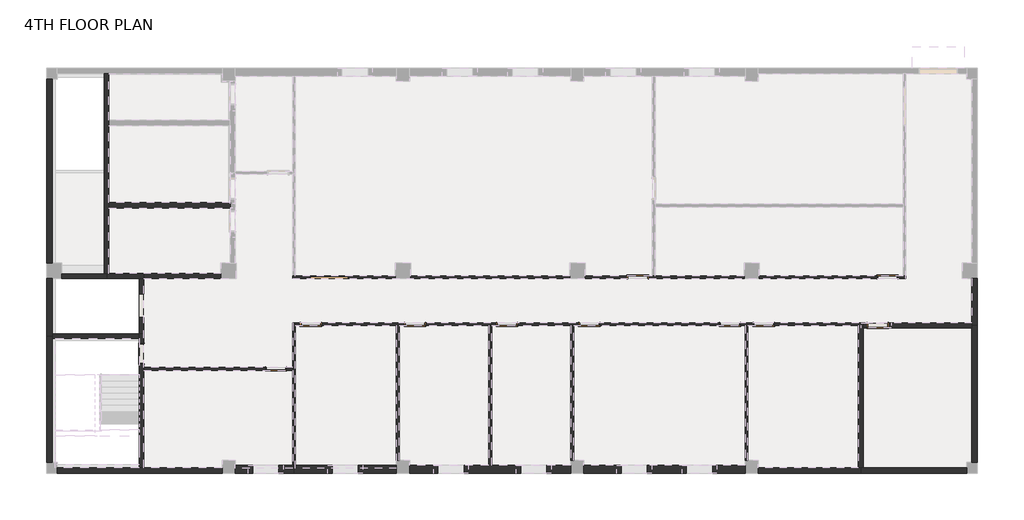
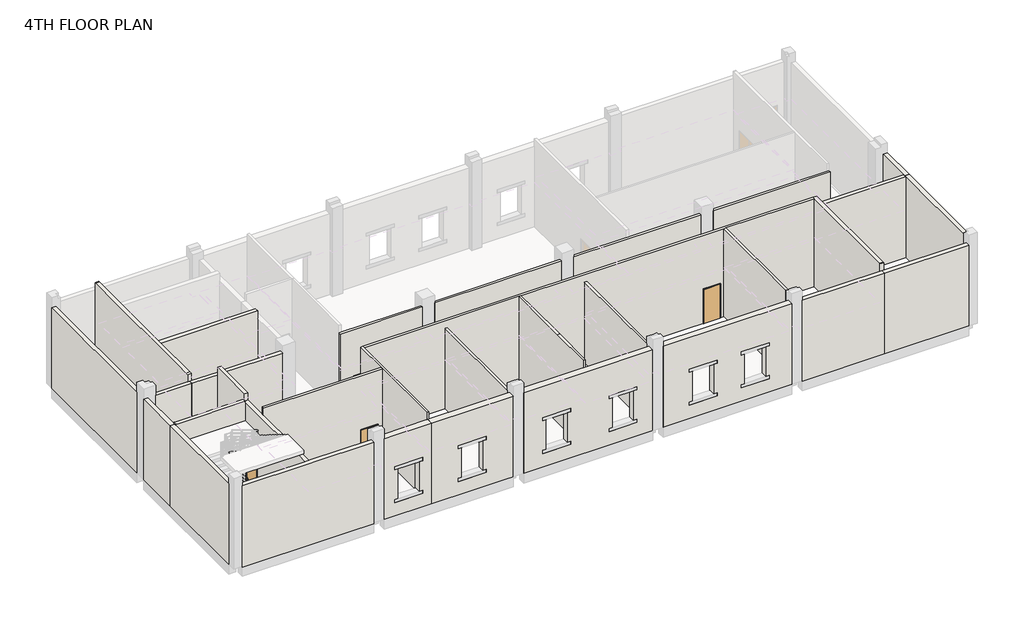
# One storey, part 1 of 6: 34 walls, 12 doors.
# Revit data of these elements (continued)
# Type "DR110-Single Door : DR111-Steel Door-1000x2100mm"
#   Description = "DSDSSD"
#   Type Mark = "SD"
#   Analytic Construction = "<None>"
#   프레임 투영 외부. = 25 mm
#   프레임 투영 내부. = 25 mm
#   프레임 폭 = 75 mm
#   Height = 2100 mm
#   Width = 1000 mm
#   Define Thermal Properties by = 1
#   문 패널 = SD1 문 패널
#   문 프레임 = A04AQ098-00002_Steel Door_non FP_single
#   Function = (empty or 0)
#   Wall Closure = (empty or 0)
# Type "DR110-Single Door : DR112-Steel Door-1000x2100mm_Panic Bar"
#   Type Mark = "SD"
#   Analytic Construction = "<None>"
#   프레임 투영 외부. = 25 mm
#   프레임 투영 내부. = 25 mm
#   프레임 폭 = 75 mm
#   Height = 2100 mm
#   Width = 1000 mm
#   Define Thermal Properties by = 1
#   문 패널 = SD1 문 패널
#   문 프레임 = A04AQ098-00002_Steel Door_non FP_single
#   Function = (empty or 0)
#   Wall Closure = (empty or 0)
# Type "DR120-Double Door : DR121-Steel Door-2000x2100mm"
#   Type Mark = "SD"
#   프레임 = ""
#   철물 = ""
#   유리/마감 = ""
#   위치/개소 = ""
#   부호 = "1/SD"
#   문번호 = ""
#   문기호 = "SD"
#   Analytic Construction = "<None>"
#   Height = 2100 mm
#   Width = 1800 mm
#   Define Thermal Properties by = 1
#   문 틀 = A04AQ098-00003_Steel Door_non FP_double
#   문 = 문
#   Function = (empty or 0)
#   Assembly Code = ""
#   Wall Closure = (empty or 0)
# Type "WA120_Ext. RC Wall_AG_300- W1(2)"
#   Type Comments = ""
#   Type Mark = "W1"
#   Layers, outside or top first: 1 mm "A04AL077-00001_Ext Wall Painting_Acrylic Emulsion Paint" (function 4); 250 mm "A03AD032-00007_Structural Concrete_25MPa-30MPa" (function 1); 0 mm "A03AD036-00001_Form Work (1 time in use)" (function 100)
# Type "WA120_Ext. RC Wall_AG_300- W1(1)"
#   Type Comments = ""
#   Type Mark = "W1"
#   Layers, outside or top first: 1 mm "A04AL077-00001_Ext Wall Painting_Acrylic Emulsion Paint" (function 4); 250 mm "A03AD032-00007_Structural Concrete_25MPa-30MPa" (function 1); 0 mm "A03AD036-00001_Form Work (1 time in use)" (function 100); 1 mm "A04AL078-00002_Int Wall Painting_Water Emulsion Paint" (function 5); 0 mm "A04AL081-00007_Skirt_Epoxy Paint" (function 100)
# Type "WA120_Ext. RC Wall_AG_300- W1(3)"
#   Type Comments = ""
#   Type Mark = "W1"
#   Layers, outside or top first: 1 mm "A04AL077-00001_Ext Wall Painting_Acrylic Emulsion Paint" (function 4); 250 mm "A03AD032-00007_Structural Concrete_25MPa-30MPa" (function 1); 0 mm "A03AD036-00001_Form Work (1 time in use)" (function 100); 1 mm "A04AL078-00002_Int Wall Painting_Water Emulsion Paint" (function 5); 0 mm "A04AM084-00013_Skirt_Vinyl Tile w/Mortar Bond Coat or Adhesive" (function 100)
# Type "WA140_Int. RC Wall_200- W2"
#   Type Comments = ""
#   Type Mark = "W2"
#   Layers, outside or top first: 200 mm "A03AD032-00007_Structural Concrete_25MPa-30MPa" (function 1)
# Type "WAFC221_Int. Brick Wall_200_7"
#   Type Comments = ""
#   Layers, outside or top first: 190 mm "A04AK073-00002_Concrete Brick_1.0B" (function 1); 0 mm "A04AN085-00001_Liquid Waterproofing" (function 100); 21 mm "A04AS164-00002_Plastering_Int" (function 2); 9 mm "A04AM082-00002_Wall Tile_Glazed ceramic tile w/Mortar Bond Coat or Adhesive" (function 5)
# Type "WAFC221_Int. Brick Wall_200_1"
#   Type Comments = ""
#   Layers, outside or top first: 0 mm "A04AL081-00002_Skirt_Epoxy Paint" (function 100); 1 mm "A04AL078-00002_Int Wall Painting_Water Emulsion Paint" (function 4); 15 mm "A04AS164-00002_Plastering_Int" (function 2); 190 mm "A04AK073-00002_Concrete Brick_1.0B" (function 1); 15 mm "A04AS164-00002_Plastering_Int" (function 2); 1 mm "A04AL078-00002_Int Wall Painting_Water Emulsion Paint" (function 5); 0 mm "A04AM084-00013_Skirt_Vinyl Tile w/Mortar Bond Coat or Adhesive" (function 100)
# Type "WAFC221_Int. Brick Wall_200_8"
#   Type Comments = ""
#   Layers, outside or top first: 9 mm "A04AM082-00002_Wall Tile_Glazed ceramic tile w/Mortar Bond Coat or Adhesive" (function 4); 21 mm "A04AS164-00002_Plastering_Int" (function 2); 0 mm "A04AN085-00001_Liquid Waterproofing" (function 100); 190 mm "A04AK073-00002_Concrete Brick_1.0B" (function 1); 0 mm "A04AN085-00001_Liquid Waterproofing" (function 100); 21 mm "A04AS164-00002_Plastering_Int" (function 2); 9 mm "A04AM082-00002_Wall Tile_Glazed ceramic tile w/Mortar Bond Coat or Adhesive" (function 5)
# Type "WAFC221_Int. Brick Wall_200_6"
#   Type Comments = ""
#   Layers, outside or top first: 0 mm "A04AM084-00013_Skirt_Vinyl Tile w/Mortar Bond Coat or Adhesive" (function 100); 1 mm "A04AL078-00002_Int Wall Painting_Water Emulsion Paint" (function 4); 15 mm "A04AS164-00002_Plastering_Int" (function 2); 190 mm "A04AK073-00002_Concrete Brick_1.0B" (function 1); 0 mm "A04AN085-00001_Liquid Waterproofing" (function 100); 21 mm "A04AS164-00002_Plastering_Int" (function 2); 9 mm "A04AM082-00002_Wall Tile_Glazed ceramic tile w/Mortar Bond Coat or Adhesive" (function 5)
# Type "WA140_Int. RC Wall_200- W2(1)"
#   Type Comments = ""
#   Type Mark = "W2"
#   Layers, outside or top first: 0 mm "A04AM084-00013_Skirt_Vinyl Tile w/Mortar Bond Coat or Adhesive" (function 100); 1 mm "A04AL078-00002_Int Wall Painting_Water Emulsion Paint" (function 4); 200 mm "A03AD032-00007_Structural Concrete_25MPa-30MPa" (function 1); 0 mm "A03AD036-00001_Form Work (1 time in use)" (function 100); 1 mm "A04AL078-00002_Int Wall Painting_Water Emulsion Paint" (function 4); 0 mm "A04AM084-00013_Skirt_Vinyl Tile w/Mortar Bond Coat or Adhesive" (function 100)
# Type "WA140_Int. RC Wall_200- W2(3)"
#   Type Comments = ""
#   Type Mark = "W2"
#   Layers, outside or top first: 200 mm "A03AD032-00007_Structural Concrete_25MPa-30MPa" (function 1); 0 mm "A03AD036-00001_Form Work (1 time in use)" (function 100); 1 mm "A04AL078-00002_Int Wall Painting_Water Emulsion Paint" (function 4); 0 mm "A04AL081-00007_Skirt_Epoxy Paint" (function 100)
# Type "WA140_Int. RC Wall_200- W2(2)"
#   Type Comments = ""
#   Type Mark = "W2"
#   Layers, outside or top first: 200 mm "A03AD032-00007_Structural Concrete_25MPa-30MPa" (function 1); 0 mm "A03AD036-00001_Form Work (1 time in use)" (function 100); 1 mm "A04AL078-00002_Int Wall Painting_Water Emulsion Paint" (function 4); 0 mm "A04AM084-00013_Skirt_Vinyl Tile w/Mortar Bond Coat or Adhesive" (function 100)
# Type "WAFC356 Interior-WF-Ceramic Tile"
#   Type Comments = ""
#   Layers, outside or top first: 0 mm "A04AN085-00001_Liquid Waterproofing" (function 100); 21 mm "A04AS164-00002_Plastering_Int" (function 2); 9 mm "A04AM082-00002_Wall Tile_Glazed ceramic tile w/Mortar Bond Coat or Adhesive" (function 4)
# Type "WA452_Int. Gypsum Wall 2 Layer_2 Hr_125"
#   Type Comments = ""
#   Layers, outside or top first: 0 mm "A04AM084-00013_Skirt_Vinyl Tile w/Mortar Bond Coat or Adhesive" (function 100); 0 mm "A04AL078-00002_Int Wall Painting_Water Emulsion Paint" (function 100); 125 mm "A04AR143-00010_Gypsumboard Partition Wall_THK 12.5mm 2ply_Mineral wool" (function 2); 0 mm "A04AL078-00002_Int Wall Painting_Water Emulsion Paint" (function 100); 0 mm "A04AM084-00013_Skirt_Vinyl Tile w/Mortar Bond Coat or Adhesive" (function 100)
# Type "WAF310_Ext. Cavity Wall Brick_90_50_190_1"
#   Type Comments = ""
#   Layers, outside or top first: 1 mm "A04AL077-00001_Ext Wall Painting_Acrylic Emulsion Paint" (function 4); 20 mm "A04AS164-00001_Plastering_Ext" (function 2); 90 mm "A04AK073-00001_Concrete Brick_0.5B" (function 1); 50 mm "A04AK076-00001_Mineral Wool_THK 50-75mm" (function 3); 190 mm "A04AK073-00002_Concrete Brick_1.0B" (function 1); 15 mm "A04AS164-00002_Plastering_Int" (function 2); 1 mm "A04AL078-00002_Int Wall Painting_Water Emulsion Paint" (function 4); 0 mm "A04AL081-00007_Skirt_Epoxy Paint" (function 100)
# Type "WAF310_Ext. Cavity Wall Brick_90_50_190_2"
#   Type Comments = ""
#   Layers, outside or top first: 1 mm "A04AL077-00001_Ext Wall Painting_Acrylic Emulsion Paint" (function 4); 20 mm "A04AS164-00001_Plastering_Ext" (function 2); 90 mm "A04AK073-00001_Concrete Brick_0.5B" (function 1); 50 mm "A04AK076-00001_Mineral Wool_THK 50-75mm" (function 3); 190 mm "A04AK073-00002_Concrete Brick_1.0B" (function 1); 15 mm "A04AS164-00002_Plastering_Int" (function 2); 1 mm "A04AL078-00002_Int Wall Painting_Water Emulsion Paint" (function 4); 0 mm "A04AM084-00013_Skirt_Vinyl Tile w/Mortar Bond Coat or Adhesive" (function 100)
# Elements 1, 2, 3, 4, 5, 6, 7, 8, 9, 10 (IfcDoor, "DR110-Single Door : DR111-Steel Door-1000x2100mm")
#   Head = "1"
#   Jamb = "2"
#   Sill = "5"
#   Door Type = "A"
#   Phase Created = New Construction
#   Materials on its faces: "A04AQ098-00002_Steel Door_non FP_single", "SD1 문 패널"
# Element 11 (IfcDoor, "DR110-Single Door : DR112-Steel Door-1000x2100mm_Panic Bar")
#   Head = "1"
#   Jamb = "2"
#   Sill = "3"
#   Door Type = "A"
#   Phase Created = New Construction
#   Materials on its faces: "A04AQ098-00002_Steel Door_non FP_single", "SD1 문 패널"
# Element 12 (IfcDoor, "DR120-Double Door : DR121-Steel Door-2000x2100mm")
#   Head = "1"
#   Jamb = "2"
#   Sill = "5"
#   Door Type = "B"
#   FLOOR = "4TH FLOOR PLAN"
#   Phase Created = New Construction
#   Materials on its faces: "A04AQ098-00003_Steel Door_non FP_double", "문"
# Element 13 (IfcWall, "WA120_Ext. RC Wall_AG_300- W1(2)")
#   Top Offset = -600 mm
#   Base Offset = 0 mm
#   wall height = 4900 mm
#   Phase Created = New Construction
#   Base Constraint = 4TH FLOOR PLAN
#   Top Constraint = ROOF PLAN
#   Materials on its faces: "Default Wall", "A04AL077-00001_Ext Wall Painting_Acrylic Emulsion Paint", "A03AD032-00007_Structural Concrete_25MPa-30MPa"
# Elements 14, 29 (IfcWall, "WA120_Ext. RC Wall_AG_300- W1(1)")
#   Top Offset = -600 mm
#   Base Offset = 0 mm
#   wall height = 4900 mm
#   Phase Created = New Construction
#   Base Constraint = 4TH FLOOR PLAN
#   Top Constraint = ROOF PLAN
#   Materials on its faces: "Default Wall", "A04AL077-00001_Ext Wall Painting_Acrylic Emulsion Paint", "A04AL078-00002_Int Wall Painting_Water Emulsion Paint"
# Element 15 (IfcWall, "WA120_Ext. RC Wall_AG_300- W1(3)")
#   Top Offset = -600 mm
#   Base Offset = 0 mm
#   wall height = 4900 mm
#   Phase Created = New Construction
#   Base Constraint = 4TH FLOOR PLAN
#   Top Constraint = ROOF PLAN
#   Materials on its faces: "Default Wall", "A04AL078-00002_Int Wall Painting_Water Emulsion Paint", "A04AL077-00001_Ext Wall Painting_Acrylic Emulsion Paint"
# Element 16 (IfcWall, "WA140_Int. RC Wall_200- W2")
#   built-in parameter 1001111 = -50 mm
#   Top Offset = -600 mm
#   Base Offset = -50 mm
#   wall height = 4950 mm
#   Phase Created = New Construction
#   Base Constraint = 4TH FLOOR PLAN
#   Top Constraint = ROOF PLAN
#   Materials on its faces: "A03AD032-00007_Structural Concrete_25MPa-30MPa", "A04AL078-00002_Int Wall Painting_Water Emulsion Paint"
# Element 17 (IfcWall, "WAFC221_Int. Brick Wall_200_7")
#   built-in parameter 1001111 = -50 mm
#   Top Offset = -150 mm
#   Base Offset = -50 mm
#   wall height = 5400 mm
#   Phase Created = New Construction
#   Base Constraint = 4TH FLOOR PLAN
#   Top Constraint = ROOF PLAN
#   Materials on its faces: "Default Wall", "A04AM082-00002_Wall Tile_Glazed ceramic tile w/Mortar Bond Coat or Adhesive", "A04AK073-00002_Concrete Brick_1.0B"
# Element 18 (IfcWall, "WAFC221_Int. Brick Wall_200_1")
#   built-in parameter 1001111 = -50 mm
#   Top Offset = -150 mm
#   Base Offset = -50 mm
#   wall height = 5400 mm
#   Phase Created = New Construction
#   Base Constraint = 4TH FLOOR PLAN
#   Top Constraint = ROOF PLAN
#   Materials on its faces: "Default Wall", "A04AL078-00002_Int Wall Painting_Water Emulsion Paint"
# Element 19 (IfcWall, "WAFC221_Int. Brick Wall_200_1")
#   built-in parameter 1001111 = -50 mm
#   Top Offset = -600 mm
#   Base Offset = -50 mm
#   wall height = 4950 mm
#   Phase Created = New Construction
#   Base Constraint = 4TH FLOOR PLAN
#   Top Constraint = ROOF PLAN
#   Materials on its faces: "Default Wall", "A04AL078-00002_Int Wall Painting_Water Emulsion Paint"
# Element 20 (IfcWall, "WAFC221_Int. Brick Wall_200_8")
#   built-in parameter 1001111 = -50 mm
#   Top Offset = -150 mm
#   Base Offset = -50 mm
#   wall height = 5400 mm
#   Phase Created = New Construction
#   Base Constraint = 4TH FLOOR PLAN
#   Top Constraint = ROOF PLAN
#   Materials on its faces: "Default Wall", "A04AM082-00002_Wall Tile_Glazed ceramic tile w/Mortar Bond Coat or Adhesive"
# Element 21 (IfcWall, "WAFC221_Int. Brick Wall_200_6")
#   Top Offset = -600 mm
#   Base Offset = 0 mm
#   wall height = 4900 mm
#   Phase Created = New Construction
#   Base Constraint = 4TH FLOOR PLAN
#   Top Constraint = ROOF PLAN
#   Materials on its faces: "Default Wall", "A04AM082-00002_Wall Tile_Glazed ceramic tile w/Mortar Bond Coat or Adhesive", "A04AL078-00002_Int Wall Painting_Water Emulsion Paint"
# Element 22 (IfcWall, "WA120_Ext. RC Wall_AG_300- W1(3)")
#   built-in parameter 1001111 = -50 mm
#   Top Offset = -600 mm
#   Base Offset = -50 mm
#   wall height = 4950 mm
#   Phase Created = New Construction
#   Base Constraint = 4TH FLOOR PLAN
#   Top Constraint = ROOF PLAN
#   Materials on its faces: "Default Wall", "A04AL077-00001_Ext Wall Painting_Acrylic Emulsion Paint", "A04AL078-00002_Int Wall Painting_Water Emulsion Paint"
# Element 23 (IfcWall, "WA120_Ext. RC Wall_AG_300- W1(1)")
#   Top Offset = -600 mm
#   Base Offset = 0 mm
#   wall height = 4900 mm
#   Phase Created = New Construction
#   Base Constraint = 4TH FLOOR PLAN
#   Top Constraint = ROOF PLAN
#   Materials on its faces: "Default Wall", "A04AL078-00002_Int Wall Painting_Water Emulsion Paint", "A04AL077-00001_Ext Wall Painting_Acrylic Emulsion Paint"
# Element 24 (IfcWall, "WA140_Int. RC Wall_200- W2(1)")
#   built-in parameter 1001111 = -50 mm
#   Top Offset = -600 mm
#   Base Offset = -50 mm
#   wall height = 4950 mm
#   Phase Created = New Construction
#   Base Constraint = 4TH FLOOR PLAN
#   Top Constraint = ROOF PLAN
#   Materials on its faces: "Default Wall", "A04AL078-00002_Int Wall Painting_Water Emulsion Paint", "A03AD032-00007_Structural Concrete_25MPa-30MPa"
# Element 25 (IfcWall, "WA140_Int. RC Wall_200- W2(3)")
#   built-in parameter 1001111 = -50 mm
#   Top Offset = -550 mm
#   Base Offset = -50 mm
#   wall height = 5000 mm
#   Phase Created = New Construction
#   Base Constraint = 4TH FLOOR PLAN
#   Top Constraint = ROOF PLAN
#   Materials on its faces: "Default Wall", "A04AL078-00002_Int Wall Painting_Water Emulsion Paint", "A03AD032-00007_Structural Concrete_25MPa-30MPa"
# Element 26 (IfcWall, "WA140_Int. RC Wall_200- W2(2)")
#   Comments = ""
#   built-in parameter 1001111 = -50 mm
#   Top Offset = -150 mm
#   Base Offset = -50 mm
#   wall height = 5400 mm
#   Phase Created = New Construction
#   Base Constraint = 4TH FLOOR PLAN
#   Top Constraint = ROOF PLAN
#   Materials on its faces: "Default Wall", "A04AL078-00002_Int Wall Painting_Water Emulsion Paint", "A03AD032-00007_Structural Concrete_25MPa-30MPa"
# Element 27 (IfcWall, "WA140_Int. RC Wall_200- W2")
#   built-in parameter 1001111 = -50 mm
#   Top Offset = -600 mm
#   Base Offset = -50 mm
#   wall height = 4950 mm
#   Phase Created = New Construction
#   Base Constraint = 4TH FLOOR PLAN
#   Top Constraint = ROOF PLAN
#   Materials on its faces: "A03AD032-00007_Structural Concrete_25MPa-30MPa"
# Element 28 (IfcWall, "WA120_Ext. RC Wall_AG_300- W1(3)")
#   Top Offset = -600 mm
#   Base Offset = 0 mm
#   wall height = 4900 mm
#   Phase Created = New Construction
#   Base Constraint = 4TH FLOOR PLAN
#   Top Constraint = ROOF PLAN
#   Materials on its faces: "Default Wall", "A04AL077-00001_Ext Wall Painting_Acrylic Emulsion Paint", "A04AL078-00002_Int Wall Painting_Water Emulsion Paint"
# Element 30 (IfcWall, "WAFC356 Interior-WF-Ceramic Tile")
#   Top Offset = 0 mm
#   Base Offset = 0 mm
#   Unconnected Height = 3000 mm
#   wall height = 3000 mm
#   Phase Created = New Construction
#   Base Constraint = 4TH FLOOR PLAN
#   Materials on its faces: "Default Wall", "A04AM082-00002_Wall Tile_Glazed ceramic tile w/Mortar Bond Coat or Adhesive", "A04AS164-00002_Plastering_Int"
# Element 31 (IfcWall, "WA120_Ext. RC Wall_AG_300- W1(2)")
#   Comments = ""
#   Top Offset = -600 mm
#   Base Offset = 0 mm
#   wall height = 4900 mm
#   Phase Created = New Construction
#   Base Constraint = 4TH FLOOR PLAN
#   Top Constraint = ROOF PLAN
#   Materials on its faces: "Default Wall", "A04AL077-00001_Ext Wall Painting_Acrylic Emulsion Paint", "A03AD032-00007_Structural Concrete_25MPa-30MPa"
# Elements 32, 36, 37, 38, 39, 40 (IfcWall, "WA452_Int. Gypsum Wall 2 Layer_2 Hr_125")
#   Top Offset = -600 mm
#   Base Offset = 0 mm
#   wall height = 4900 mm
#   Phase Created = New Construction
#   Base Constraint = 4TH FLOOR PLAN
#   Top Constraint = ROOF PLAN
#   Materials on its faces: "Default Wall", "A04AR143-00010_Gypsumboard Partition Wall_THK 12.5mm 2ply_Mineral wool"
# Elements 33, 34, 35, 42 (IfcWall, "WA452_Int. Gypsum Wall 2 Layer_2 Hr_125")
#   Top Offset = -150 mm
#   Base Offset = 0 mm
#   wall height = 5350 mm
#   Phase Created = New Construction
#   Base Constraint = 4TH FLOOR PLAN
#   Top Constraint = ROOF PLAN
#   Materials on its faces: "Default Wall", "A04AR143-00010_Gypsumboard Partition Wall_THK 12.5mm 2ply_Mineral wool"
# Element 41 (IfcWall, "WA452_Int. Gypsum Wall 2 Layer_2 Hr_125")
#   Top Offset = -150 mm
#   Base Offset = 0 mm
#   wall height = 5350 mm
#   Phase Created = New Construction
#   Base Constraint = 4TH FLOOR PLAN
#   Top Constraint = ROOF PLAN
#   Materials on its faces: "A04AR143-00010_Gypsumboard Partition Wall_THK 12.5mm 2ply_Mineral wool", "Default Wall"
# Element 43 (IfcWall, "WAF310_Ext. Cavity Wall Brick_90_50_190_1")
#   Top Offset = -600 mm
#   Base Offset = 0 mm
#   wall height = 4900 mm
#   Phase Created = New Construction
#   Base Constraint = 4TH FLOOR PLAN
#   Top Constraint = ROOF PLAN
#   Materials on its faces: "Default Wall", "A04AL077-00001_Ext Wall Painting_Acrylic Emulsion Paint", "A04AL078-00002_Int Wall Painting_Water Emulsion Paint"
# Elements 44, 45, 46 (IfcWall, "WAF310_Ext. Cavity Wall Brick_90_50_190_2")
#   Top Offset = -600 mm
#   Base Offset = 0 mm
#   wall height = 4900 mm
#   Phase Created = New Construction
#   Base Constraint = 4TH FLOOR PLAN
#   Top Constraint = ROOF PLAN
#   Materials on its faces: "Default Wall", "A04AL077-00001_Ext Wall Painting_Acrylic Emulsion Paint", "A04AL078-00002_Int Wall Painting_Water Emulsion Paint"
# Materials
#   "SD1 문 패널": class "금속", colour RGB 247 247 247, transparency 0, Description = "STEEL DOOR (1000Wx2100H)"
#   "A04AQ098-00002_Steel Door_non FP_single": class "금속", colour RGB 247 247 247, transparency 0, Description = "Steel Door", W00) Work Master Code = "A04AQ098-00002", W01) Work Master_Lv1 = "Finishing Work", W02) Work Master_Lv2 = "Door & Window Work", W03) Work Master_Spec.1 = "Steel Door w/ Steel Frame", W04) Work Master_Spec.2 = "Fire Protective Rating: N/A, Single Door", W05) Work Master_Spec.3 = "w/ Hardware & Accessories", Cost = 0
#   "A04AQ098-00003_Steel Door_non FP_double": class "금속", colour RGB 247 247 247, transparency 0, Description = "Steel Door", W00) Work Master Code = "A04AQ098-00003", W01) Work Master_Lv1 = "Finishing Work", W02) Work Master_Lv2 = "Door & Window Work", W03) Work Master_Spec.1 = "Steel Door w/ Steel Frame", W04) Work Master_Spec.2 = "Fire Protective Rating: N/A, Double Door", W05) Work Master_Spec.3 = "w/ Hardware & Accessories", Cost = 0
#   "문": class "다양한", colour RGB 247 247 247, transparency 0
#   "A04AL077-00001_Ext Wall Painting_Acrylic Emulsion Paint": class "Finish", colour RGB 128 128 64, transparency 0, Description = "ACRYLIC EMULSION PAINT", W00) Work Master Code = "A04AL077-00001", W01) Work Master_Lv1 = "Finishing Work", W02) Work Master_Lv2 = "Painting Work", W03) Work Master_Spec.1 = "External Wall Painting", W04) Work Master_Spec.2 = "Acrylic Emulsion Paint", Cost = 0
#   "A03AD032-00007_Structural Concrete_25MPa-30MPa": class "Concrete", colour RGB 176 176 176, transparency 0, Keynote = "09910.A1", Description = "ACRYLIC EMULSION PAINT ON\nFAIR FACED CONC.", W00) Work Master Code = "A03AD032-00007", W01) Work Master_Lv1 = "Concrete Work", W02) Work Master_Lv2 = "Superstructure Work", W03) Work Master_Spec.1 = "Structural Concrete", W04) Work Master_Spec.2 = "Cement Type-1", W05) Work Master_Spec.3 = "25MPa < F'c (Cylinder Strength) ≤ 30MPa", Cost = 0
#   "A03AD036-00001_Form Work (1 time in use)": class "Wood", colour RGB 149 120 74, transparency 0, Description = "Plywood", W00) Work Master Code = "A03AD036-00001", W01) Work Master_Lv1 = "Concrete Work", W02) Work Master_Lv2 = "Superstructure Work", W03) Work Master_Spec.1 = "Form Work (1 time in use)", W04) Work Master_Spec.2 = "Flat Form", W05) Work Master_Spec.3 = "Dressed Lumber, Plywood or Steel Form(Wood Planks are not Allowed) incl. Chamfer", Cost = 0
#   "A04AL078-00002_Int Wall Painting_Water Emulsion Paint": class "Finish", colour RGB 128 128 64, transparency 0, Description = "WATER EMULSION PAINT", W00) Work Master Code = "A04AL078-00002", W01) Work Master_Lv1 = "Finishing Work", W02) Work Master_Lv2 = "Painting Work", W03) Work Master_Spec.1 = "Internal Wall Painting", W04) Work Master_Spec.2 = "Water Emulsion Paint", Cost = 0
#   "A04AL081-00007_Skirt_Epoxy Paint": class "Finish", colour RGB 128 128 64, transparency 0, Description = "플라스틱", W00) Work Master Code = "A04AL081-00007", W01) Work Master_Lv1 = "Finishing Work", W02) Work Master_Lv2 = "Painting Work", W03) Work Master_Spec.1 = "Skirt Painting", W04) Work Master_Spec.2 = "Epoxy Paint", W05) Work Master_Spec.3 = "100mm≤H<150mm", Cost = 0
#   "A04AM084-00013_Skirt_Vinyl Tile w/Mortar Bond Coat or Adhesive": class "Plastic", colour RGB 244 237 124, transparency 0, Description = "플렉시블 폴리 염화 비닐", W00) Work Master Code = "A04AM084-00013", W01) Work Master_Lv1 = "Finishing Work", W02) Work Master_Lv2 = "Tile Work", W03) Work Master_Spec.1 = "Skirt Painting", W04) Work Master_Spec.2 = "Vinyl Tile", W05) Work Master_Spec.3 = "w/ Mortar Bond Coat or Adhesive", Cost = 0
#   "A04AK073-00002_Concrete Brick_1.0B": class "Concrete", colour RGB 180 180 180, transparency 0, Description = "THK.190 CONC. BLOCK", W00) Work Master Code = "A04AK073-00002", W01) Work Master_Lv1 = "Finishing Work", W02) Work Master_Lv2 = "Masonry Work", W03) Work Master_Spec.1 = "Concrete Brick", W04) Work Master_Spec.2 = "[1.0B] w/ All Reinf.(Lath, Steel Tie, Anchor Bar, Mortar, ETC.), Filler, Sealant, Lintel/Sill for Opening, ETC.", Cost = 0
#   "A04AN085-00001_Liquid Waterproofing": class "Plastic", colour RGB 127 127 127, transparency 0, Description = "Exterior finish, roofing", W00) Work Master Code = "A04AN085-00001", W01) Work Master_Lv1 = "Finishing Work", W02) Work Master_Lv2 = "Waterproofing Work", W03) Work Master_Spec.1 = "Liquid Waterproofing", W04) Work Master_Spec.2 = "for Internal Floor Area", W05) Work Master_Spec.3 = "Min. 2 Coats", Cost = 0
#   "A04AS164-00002_Plastering_Int": class "Concrete", colour RGB 183 186 184, transparency 0, Description = "LATEX PAINT ON THK.15 CEMENT PLASTER", W00) Work Master Code = "A04AS164-00002", W01) Work Master_Lv1 = "Finishing Work", W02) Work Master_Lv2 = "Plastering Work", W03) Work Master_Spec.1 = "Plastering", W04) Work Master_Spec.2 = "for Internal Masonry Wall", Cost = 0
#   "A04AM082-00002_Wall Tile_Glazed ceramic tile w/Mortar Bond Coat or Adhesive": class "Finish", colour RGB 245 245 245, transparency 0, Description = "Ceramic Tile", W00) Work Master Code = "A04AM082-6027", W01) Work Master_Lv1 = "Finishing Work", W02) Work Master_Lv2 = "Tile Work", W03) Work Master_Spec.1 = "Wall Tile", W04) Work Master_Spec.2 = "Glazed Ceramic Tile", W05) Work Master_Spec.3 = "w/ Mortar Bond Coat or Adhesive", Cost = 0
#   "A04AL081-00002_Skirt_Epoxy Paint": class "Finish", colour RGB 128 128 64, transparency 0, Description = "플라스틱", Cost = 0
#   "A04AR143-00010_Gypsumboard Partition Wall_THK 12.5mm 2ply_Mineral wool": class "Finish", colour RGB 171 170 168, transparency 0, Description = "Gypsum Board", W00) Work Master Code = "A04AR143-00008", W01) Work Master_Lv1 = "Finishing Work", W02) Work Master_Lv2 = "Exterior/Interior Finish Work", W03) Work Master_Spec.1 = "Gypsumboard Partition Wall (Fixed Type)", W04) Work Master_Spec.2 = "Fire Protective Rating: 2_hrs, 2-Layer Gypsum Board to Both Sides", W05) Work Master_Spec.3 = "Mineral Wool Thk.=50mm", W06) Work Master_Spec.4 = "2-Layer Gypsumboard THK=12.5mm", Cost = 0
#   "A04AS164-00001_Plastering_Ext": class "Concrete", colour RGB 183 186 184, transparency 0, Description = "ACRYLIC EMULSION PAINT ON\nCEMENT PLASTER", W00) Work Master Code = "A04AS164-00001", W01) Work Master_Lv1 = "Finishing Work", W02) Work Master_Lv2 = "Plastering Work", W03) Work Master_Spec.1 = "Plastering", W04) Work Master_Spec.2 = "for External Masonry Wall", Cost = 0
#   "A04AK073-00001_Concrete Brick_0.5B": class "Concrete", colour RGB 180 180 180, transparency 0, Description = "Conc. Block", W00) Work Master Code = "A04AK073-00001", W01) Work Master_Lv1 = "Finishing Work", W02) Work Master_Lv2 = "Masonry Work", W03) Work Master_Spec.1 = "Concrete Brick", W04) Work Master_Spec.2 = "[0.5B] w/ All Reinf.(Lath, Steel Tie, Anchor Bar, Mortar, ETC.), Filler, Sealant, Lintel/Sill for Opening, ETC.", Cost = 0
#   "A04AK076-00001_Mineral Wool_THK 50-75mm": class "Insulation", colour RGB 255 255 217, transparency 0, Description = "Insulation(Rigid)", W00) Work Master Code = "A04AK076-00001", W01) Work Master_Lv1 = "Finishing Work", W02) Work Master_Lv2 = "Masonry Work", W03) Work Master_Spec.1 = "Insulation", W04) Work Master_Spec.2 = "Mineral Wool", W05) Work Master_Spec.3 = "Minimum Density of 50 kg/m3", W06) Work Master_Spec.4 = "50mm≤THK<75mm", Cost = 0
#   "Default Wall": class "Miscellaneous", colour RGB 80 80 80, transparency 0
# Room at (33720.402, 31696.623) mm, phase "New Construction", upper level "4TH FLOOR PLAN", upper offset 2700 mm, lower offset 0 mm
#   Comments = ""
#   Base Finish = "VINYL TILE"
#   Ceiling Finish = "ACOUSTIC TILED CEILING(M-BAR)"
#   Wall Finish = "WATER EMULSION PAINT"
#   Floor Finish = "VINYL TILE W/MORTAR BOND COAT OR ADHESIVE"
#   Number = "403"
#   Name = "DOCUMENT ROOM"
#   S01) Room Name = ""
#   S02) Room Number(Project) = ""
# Room at (7261.202, 23350.111) mm, phase "New Construction", upper level "4TH FLOOR PLAN", upper offset 3000 mm, lower offset 0 mm
#   Comments = ""
#   Base Finish = "VINYL TILE"
#   Ceiling Finish = "ACOUSTIC TILED CEILING(M-BAR)"
#   Wall Finish = "WATER EMULSION PAINT"
#   Floor Finish = "VINYL TILE W/MORTAR BOND COAT OR ADHESIVE"
#   Number = "404"
#   Name = "BREAK ROOM"
#   S01) Room Name = ""
#   S02) Room Number(Project) = ""
# Room at (13324.607, 24397.611) mm, phase "New Construction", upper level "4TH FLOOR PLAN", upper offset 3000 mm, lower offset 0 mm
#   Comments = ""
#   Base Finish = "VINYL TILE"
#   Ceiling Finish = "ACOUSTIC TILED CEILING(M-BAR)"
#   Wall Finish = "WATER EMULSION PAINT"
#   Floor Finish = "VINYL TILE W/MORTAR BOND COAT OR ADHESIVE"
#   Number = "405"
#   Name = "STORAGE"
#   S01) Room Name = ""
#   S02) Room Number(Project) = ""
# Room at (18029.543, 24397.611) mm, phase "New Construction", upper level "4TH FLOOR PLAN", upper offset 3000 mm, lower offset 0 mm
#   Comments = ""
#   Base Finish = "VINYL TILE"
#   Ceiling Finish = "ACOUSTIC TILED CEILING(M-BAR)"
#   Wall Finish = "WATER EMULSION PAINT"
#   Floor Finish = "VINYL TILE W/MORTAR BOND COAT OR ADHESIVE"
#   Number = "406"
#   Name = "MANAGER ROOM-1"
#   S01) Room Name = ""
#   S02) Room Number(Project) = ""
# Room at (21959.913, 24397.611) mm, phase "New Construction", upper level "4TH FLOOR PLAN", upper offset 3000 mm, lower offset 0 mm
#   Comments = ""
#   Base Finish = "VINYL TILE"
#   Ceiling Finish = "ACOUSTIC TILED CEILING(M-BAR)"
#   Wall Finish = "WATER EMULSION PAINT"
#   Floor Finish = "VINYL TILE W/MORTAR BOND COAT OR ADHESIVE"
#   Number = "407"
#   Name = "MANAGER ROOM-2"
#   S01) Room Name = ""
#   S02) Room Number(Project) = ""
# Room at (27923.917, 24397.611) mm, phase "New Construction", upper level "4TH FLOOR PLAN", upper offset 3000 mm, lower offset 0 mm
#   Comments = ""
#   Base Finish = "VINYL TILE"
#   Ceiling Finish = "ACOUSTIC TILED CEILING(M-BAR)"
#   Wall Finish = "WATER EMULSION PAINT"
#   Floor Finish = "VINYL TILE W/MORTAR BOND COAT OR ADHESIVE"
#   Number = "408"
#   Name = "MEETING ROOM-2"
#   S01) Room Name = ""
#   S02) Room Number(Project) = ""
# Room at (34795.021, 24350.111) mm, phase "New Construction", upper level "4TH FLOOR PLAN", upper offset 3000 mm, lower offset 0 mm
#   Comments = ""
#   Base Finish = "VINYL TILE"
#   Ceiling Finish = "ACOUSTIC TILED CEILING(M-BAR)"
#   Wall Finish = "WATER EMULSION PAINT"
#   Floor Finish = "VINYL TILE W/MORTAR BOND COAT OR ADHESIVE"
#   Number = "409"
#   Name = "OFFICE-1"
#   S01) Room Name = ""
#   S02) Room Number(Project) = ""
# Room at (37677.623, 23118.178) mm, phase "New Construction", upper level "4TH FLOOR PLAN", upper offset 5350 mm, lower offset 0 mm
#   Comments = ""
#   Base Finish = "EPOXY PAINT"
#   Ceiling Finish = "WATER EMULSOIN PAINT"
#   Wall Finish = "WATER EMULSION PAINT"
#   Floor Finish = "EPOXY PAINT ON STEEL TROWEL FINISH"
#   Number = "410"
#   Name = "FIRE GAS ROOM"
#   S01) Room Name = ""
#   S02) Room Number(Project) = ""
# Room at (19051.406, 34520.324) mm, phase "New Construction", upper level "4TH FLOOR PLAN", upper offset 2700 mm, lower offset 0 mm
#   Comments = ""
#   Base Finish = "VINYL TILE"
#   Ceiling Finish = "ACOUSTIC TILED CEILING(M-BAR)"
#   Wall Finish = "WATER EMULSION PAINT"
#   Floor Finish = "VINYL TILE W/MORTAR BOND COAT OR ADHESIVE"
#   Number = "401"
#   Name = "OPEN OFFICE"
#   S01) Room Name = ""
#   S02) Room Number(Project) = ""
#   FLOOR LEVEL = "4TH FLOOR PLAN"
# Room at (33720.402, 36493.41) mm, phase "New Construction", upper level "4TH FLOOR PLAN", upper offset 3000 mm, lower offset 0 mm
#   Comments = ""
#   Base Finish = "VINYL TILE"
#   Ceiling Finish = "ACOUSTIC TILED CEILING(M-BAR)"
#   Wall Finish = "WATER EMULSION PAINT"
#   Floor Finish = "VINYL TILE W/MORTAR BOND COAT OR ADHESIVE"
#   Number = "402"
#   Name = "MEETING ROOM-1"
#   S01) Room Name = ""
#   S02) Room Number(Project) = ""
# Room at (4929.218, 38076.999) mm, phase "New Construction", upper level "4TH FLOOR PLAN", upper offset 2800 mm, lower offset 0 mm
#   Comments = ""
#   Base Finish = "-"
#   Ceiling Finish = "MOISTURE RESISTANT TILE CEILING(M-BAR)"
#   Wall Finish = "GLAZED CERAMIC TILE W/WATERPROOFING"
#   Floor Finish = "NON SLIP CERAMIC TILE ON CEMENT MORTAR W/WATERPROOFING"
#   Number = "411"
#   Name = "SHOWER ROOM(M)"
#   S01) Room Name = ""
#   S02) Room Number(Project) = ""
# Room at (4929.218, 35005.212) mm, phase "New Construction", upper level "4TH FLOOR PLAN", upper offset 2800 mm, lower offset 0 mm
#   Comments = ""
#   Base Finish = "-"
#   Ceiling Finish = "MOISTURE RESISTANT TILE CEILING(M-BAR)"
#   Wall Finish = "GLAZED CERAMIC TILE W/WATERPROOFING"
#   Floor Finish = "NON SLIP CERAMIC TILE ON CEMENT MORTAR W/WATERPROOFING"
#   Number = "413"
#   Name = "TOLITE(M)"
#   S01) Room Name = ""
#   S02) Room Number(Project) = ""
# Room at (4929.218, 31432.354) mm, phase "New Construction", upper level "4TH FLOOR PLAN", upper offset 2700 mm, lower offset 0 mm
#   Comments = ""
#   Base Finish = "-"
#   Ceiling Finish = "MOISTURE RESISTANT TILE CEILING(M-BAR)"
#   Wall Finish = "GLAZED CERAMIC TILE W/WATERPROOFING"
#   Floor Finish = "NON SLIP CERAMIC TILE ON CEMENT MORTAR W/WATERPROOFING"
#   Number = "414"
#   Name = "TOILET(F)"
#   S01) Room Name = ""
#   S02) Room Number(Project) = ""
# Room at (9614.219, 36735.303) mm, phase "New Construction", upper level "4TH FLOOR PLAN", upper offset 3000 mm, lower offset -500 mm
#   Comments = ""
#   Base Finish = "PVC VINYL TILE"
#   Ceiling Finish = "ACOUSTIC TILED CEILING(M-BAR)"
#   Wall Finish = "WATER EMULSION PAINT"
#   Floor Finish = "VINYL TILE W/MORTAR BOND COAT OR ADHESIVE"
#   Number = "412"
#   Name = "LOCKER(M)"
#   S01) Room Name = ""
#   S02) Room Number(Project) = ""
# Room at (28857.091, 28721.847) mm, phase "New Construction", upper level "4TH FLOOR PLAN", upper offset 2700 mm, lower offset 0 mm
#   Comments = ""
#   Base Finish = "PVC VINYL TILE"
#   Ceiling Finish = "ACOUSTIC TILED CEILING(M-BAR)"
#   Wall Finish = "WATER EMULSION PAINT"
#   Floor Finish = "VINYL TILE W/MORTAR BOND COAT OR ADHESIVE"
#   Number = "415"
#   Name = "CORRIDOR"
#   S01) Room Name = ""
#   S02) Room Number(Project) = ""
# Room at (1931.109, 21754.727) mm, phase "New Construction", upper level "4TH FLOOR PLAN", upper offset 2000 mm, lower offset 0 mm
#   Comments = ""
#   Base Finish = "PVC VINYL TILE"
#   Ceiling Finish = "WATER EMULSOIN PAINT"
#   Wall Finish = "WATER EMULSION PAINT"
#   Floor Finish = "VINYL TILE W/MORTAR BOND COAT OR ADHESIVE"
#   Number = "416"
#   Name = "STAIR-1"
#   S01) Room Name = ""
#   S02) Room Number(Project) = ""
